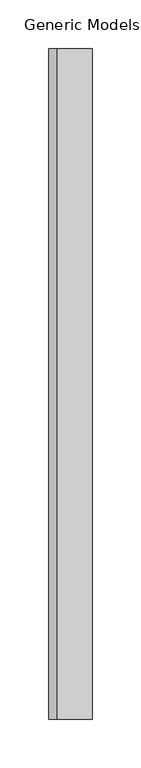
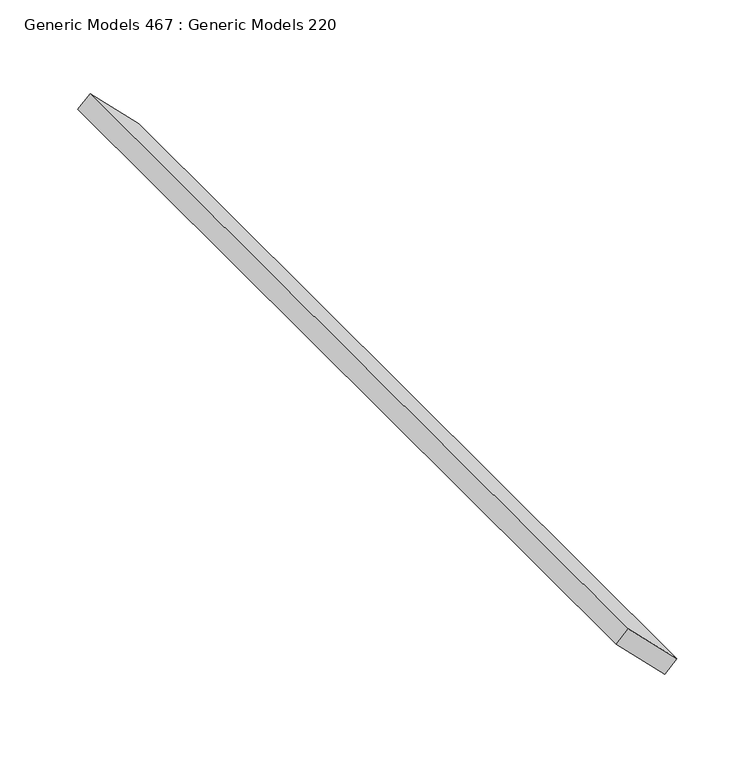
"""IFC4 building model written with IfcOpenShell, lengths in millimetres: proxy geometry, Generic Models 467 : Generic Models 220."""

from ifc_helpers import new_model, si_unit, frame, origin, place, context, project, spatial, polyline, outline, extrude, source, transform, mapped, element, save


def generic_models_467_generic_models_220_66699b01(model_context):
    return source(origin(), model_context, "Body", "SweptSolid", [
        extrude(outline(polyline([(0.0, -50.8), (0.0, 0.0), (690.8142348, 0.0), (690.8142348, -50.8), (0.0, -50.8)])), frame((-6899.085451, -4564.8872686, 128259.6762561), z_axis=(0.7071067811865582, 0.0, 0.7071067811865369), x_axis=(0.0, 1.0, 0.0)), (0.0, 0.0, 1.0), 12.7),
    ])


if __name__ == "__main__":
    model = new_model("IFC4")
    model_context = context("Model", 3, world=origin())
    ifc_project = project(units=[si_unit("LENGTHUNIT", "METRE", prefix="MILLI")], contexts=[model_context])
    site = spatial("IfcSite", under=ifc_project)
    building = spatial("IfcBuilding", under=site)
    placement = place(None, origin())
    generic_models_467_generic_models_220_shape = generic_models_467_generic_models_220_66699b01(model_context)
    element("IfcBuildingElementProxy", 1, Name="Generic Models 467 : Generic Models 220", ObjectType="Generic Models 467 : Generic Models 220", at=placement, inside=building, context=model_context, shape_type="MappedRepresentation", body=[
        mapped(generic_models_467_generic_models_220_shape, transform((0.0, 0.0, 0.0), x_axis=(1.0, 0.0, 0.0), y_axis=(0.0, 1.0, 0.0), z_axis=(0.0, 0.0, 1.0))),
    ])
    save(model, "model.ifc")

# Revit data of these elements
# Element 1 (IfcBuildingElementProxy, "Generic Models 467 : Generic Models 220")
#   Materials on its faces: "_WOOD TONE ALUMINUM EXTRUSION SLAT BY KNOTWOOD"
# Materials
#   "_WOOD TONE ALUMINUM EXTRUSION SLAT BY KNOTWOOD": class "Generic", colour RGB 177 130 114, transparency 0, Cost = 0
